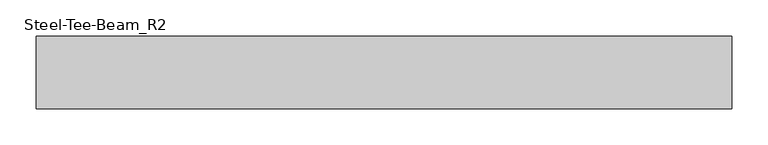
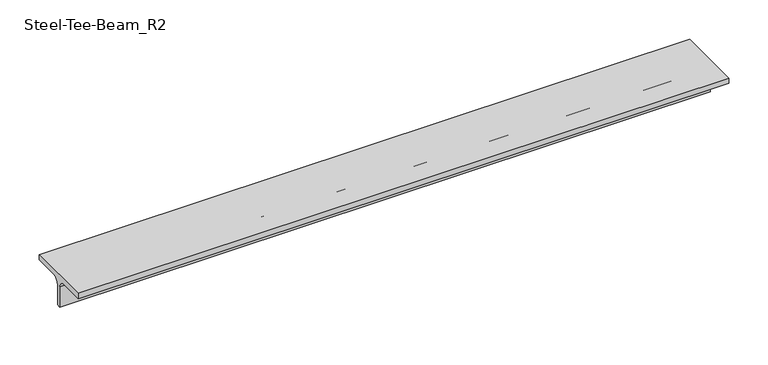
"""IFC4 building model written with IfcOpenShell, lengths in millimetres: beam geometry, Steel-Tee-Beam_R2 : BM127_CT-50x100x6x8_TB1."""

from ifc_helpers import new_model, si_unit, point, frame, frame_2d, origin, place, context, project, spatial, polyline, circle_curve, trimmed, segment, composite_curve, outline, extrude, source, transform, mapped, element, save


def steel_tee_beam_r2_b2c95b6f(model_context):
    return source(origin(), model_context, "Body", "SweptSolid", [
        extrude(outline(composite_curve([segment(polyline([(-50.0, 25.0), (50.0, 25.0), (50.0, 17.0), (13.0, 17.0)]), True, "CONTINUOUS"), segment(trimmed(circle_curve(frame_2d((13.0, 7.0)), 10.0), [point((13.0, 17.0))], [point((3.0, 7.0))], True, "CARTESIAN"), True, "CONTINUOUS"), segment(polyline([(3.0, 7.0), (3.0, -25.0), (-3.0, -25.0), (-3.0, 7.0)]), True, "CONTINUOUS"), segment(trimmed(circle_curve(frame_2d((-13.0, 7.0)), 10.0), [point((-3.0, 7.0))], [point((-13.0, 17.0))], True, "CARTESIAN"), True, "CONTINUOUS"), segment(polyline([(-13.0, 17.0), (-50.0, 17.0), (-50.0, 25.0)]), True, "CONTINUOUS")], self_intersect=False)), frame((-480.0, 0.0, 0.0), z_axis=(1.0, 0.0, 0.0), x_axis=(0.0, 1.0, 0.0)), (0.0, 0.0, 1.0), 960.0),
    ])


if __name__ == "__main__":
    model = new_model("IFC4")
    model_context = context("Model", 3, world=origin())
    ifc_project = project(units=[si_unit("LENGTHUNIT", "METRE", prefix="MILLI")], contexts=[model_context])
    site = spatial("IfcSite", under=ifc_project)
    building = spatial("IfcBuilding", under=site)
    placement = place(None, origin())
    steel_tee_beam_r2_shape = steel_tee_beam_r2_b2c95b6f(model_context)
    element("IfcBeam", 1, ObjectType="Steel-Tee-Beam_R2 : BM127_CT-50x100x6x8_TB1", at=placement, inside=building, context=model_context, shape_type="MappedRepresentation", body=[
        mapped(steel_tee_beam_r2_shape, transform((0.0, 0.0, 0.0), x_axis=(1.0, 0.0, 0.0), y_axis=(0.0, 1.0, 0.0), z_axis=(0.0, 0.0, 1.0))),
    ])
    save(model, "model.ifc")

# Revit data of these elements
# Type "Steel-Tee-Beam_R2 : BM127_CT-50x100x6x8_TB1"
#   SteelWeight = "Light"
#   Surface Area = 0.291416 m²/m
#   Section Area = 10.9492 cm²
#   Mass per Unit Length = 8.59512 kg/m
#   Length [instance default] = 1524 mm
#   bf = 100 mm
#   d = 50 mm
#   k = 18 mm
#   r = 10 mm
#   tf = 8 mm
#   tw = 6 mm
#   hec_material4 [instance default] = none
#   hec_material3 [instance default] = none
#   hec_material2 [instance default] = none
#   hec_material1 [instance default] = none
#   Structural Material [instance default] = Steel, 45-345
#   Assembly Code = ""
# Element 1 (IfcBeam, "Steel-Tee-Beam_R2 : BM127_CT-50x100x6x8_TB1")
#   Materials on its faces: "Steel, 45-345"
# Materials
#   "Steel, 45-345": class "Metal", colour RGB 189 187 185, transparency 0, Description = "Steel 345 MPa", Cost = 0
